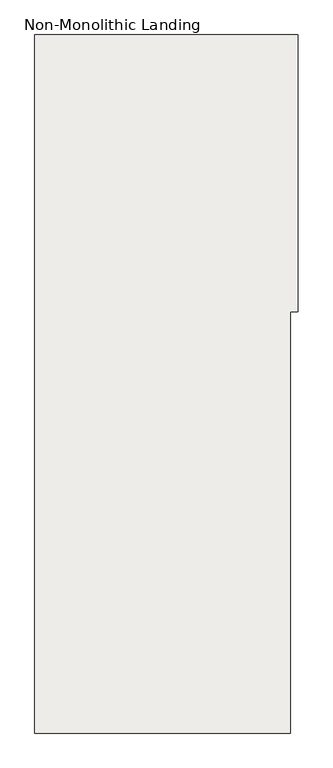
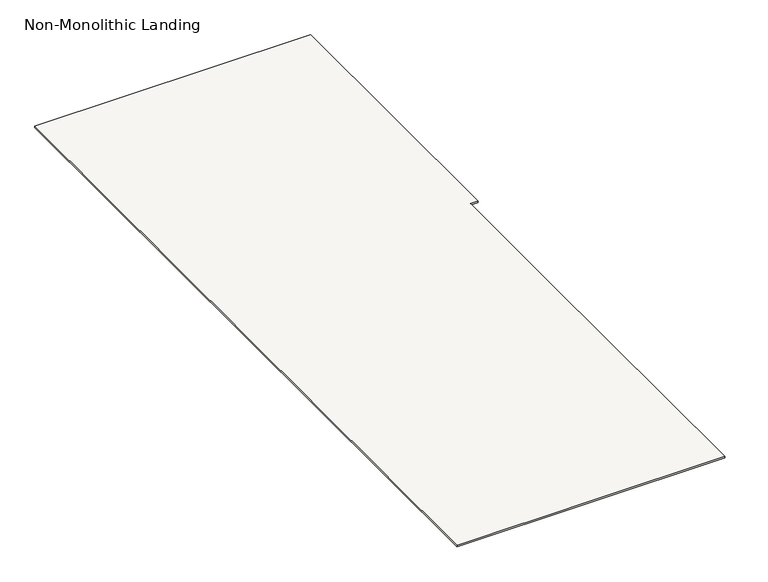
"""IFC4 building model written with IfcOpenShell, lengths in millimetres: slab geometry, Non-Monolithic Landing."""

from ifc_helpers import new_model, si_unit, origin, place, context, project, spatial, faceted_brep, source, transform, mapped, element, save


def non_monolithic_landing_0e94f8d9(model_context):
    return source(origin(), model_context, "Body", "Brep", [
        faceted_brep([(-16318.9409643, 12030.4345331, 6222.2222222), (-16318.0972143, 12030.4345331, 6216.2222222), (-16318.0972143, 13220.4345331, 6216.2222222), (-16318.9409643, 13220.4345331, 6222.2222222), (-16350.0, 11470.4345331, 6222.2222222), (-16350.0, 12030.4345331, 6222.2222222), (-16350.0, 13220.4345331, 6222.2222222), (-17450.0, 13220.4345331, 6222.2222222), (-17450.0, 10220.4345331, 6222.2222222), (-16350.0, 10220.4345331, 6222.2222222), (-16350.0, 12030.4345331, 6216.2222222), (-16350.0, 11470.4345331, 6216.2222222), (-16350.84375, 11470.4345331, 6216.2222222), (-16350.84375, 10220.4345331, 6216.2222222), (-17450.0, 10220.4345331, 6216.2222222), (-17450.0, 13220.4345331, 6216.2222222), (-16350.0, 13220.4345331, 6216.2222222)], [[[0, 1, 2, 3]], [[4, 5, 0, 3, 6, 7, 8, 9]], [[10, 11, 12, 13, 14, 15, 16, 2, 1]], [[5, 4, 11, 10]], [[0, 5, 10, 1]], [[6, 3, 2, 16]], [[7, 6, 16, 15]], [[8, 7, 15, 14]], [[9, 8, 14, 13]], [[4, 12, 11]], [[12, 4, 9, 13]]]),
    ])


if __name__ == "__main__":
    model = new_model("IFC4")
    model_context = context("Model", 3, world=origin())
    ifc_project = project(units=[si_unit("LENGTHUNIT", "METRE", prefix="MILLI")], contexts=[model_context])
    site = spatial("IfcSite", under=ifc_project)
    building = spatial("IfcBuilding", under=site)
    placement = place(None, origin())
    non_monolithic_landing_shape = non_monolithic_landing_0e94f8d9(model_context)
    element("IfcSlab", 1, ObjectType="Non-Monolithic Landing", at=placement, inside=building, context=model_context, shape_type="MappedRepresentation", body=[
        mapped(non_monolithic_landing_shape, transform((0.0, 0.0, 0.0), x_axis=(1.0, 0.0, 0.0), y_axis=(0.0, 1.0, 0.0), z_axis=(0.0, 0.0, 1.0))),
    ])
    save(model, "model.ifc")

# Revit data of these elements
# Element 1 (IfcSlab, "Non-Monolithic Landing")
#   Materials on its faces: "Steel, Paint Finish, Dark Gray"
# Materials
#   "Steel, Paint Finish, Dark Gray": class "Metal", colour RGB 89 89 89, transparency 0, Description = "Steel, paint finish, dark gray, glossy", Cost = 0
